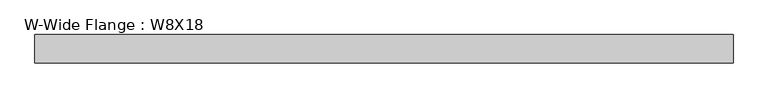
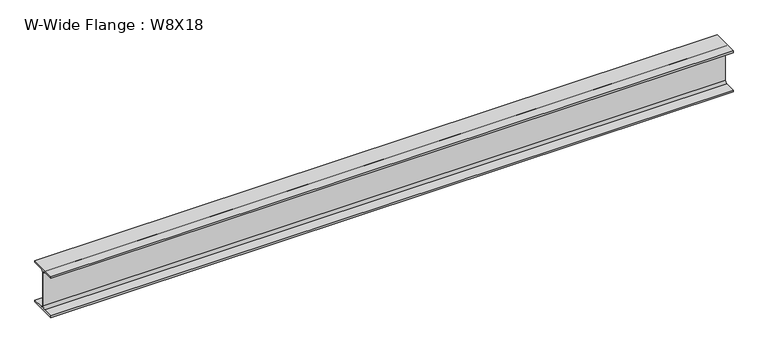
"""IFC4 building model written with IfcOpenShell, lengths in millimetres: beam geometry, W-Wide Flange : W8X18."""

from ifc_helpers import new_model, si_unit, point, frame, frame_2d, origin, place, context, project, spatial, polyline, circle_curve, trimmed, segment, composite_curve, outline, extrude, source, transform, mapped, element, save


def w_wide_flange_w8x18_c4c3ec7c(model_context):
    return source(origin(), model_context, "Body", "SweptSolid", [
        extrude(outline(composite_curve([segment(polyline([(66.675, -94.996), (66.675, -103.378), (-66.675, -103.378), (-66.675, -94.996), (-15.1765, -94.996)]), True, "CONTINUOUS"), segment(trimmed(circle_curve(frame_2d((-15.1765, -82.7405)), 12.2555), [point((-15.1765, -94.996))], [point((-2.921, -82.7405))], True, "CARTESIAN"), True, "CONTINUOUS"), segment(polyline([(-2.921, -82.7405), (-2.921, 82.7405)]), True, "CONTINUOUS"), segment(trimmed(circle_curve(frame_2d((-15.1765, 82.7405)), 12.2555), [point((-2.921, 82.7405))], [point((-15.1765, 94.996))], True, "CARTESIAN"), True, "CONTINUOUS"), segment(polyline([(-15.1765, 94.996), (-66.675, 94.996), (-66.675, 103.378), (66.675, 103.378), (66.675, 94.996), (15.1765, 94.996)]), True, "CONTINUOUS"), segment(trimmed(circle_curve(frame_2d((15.1765, 82.7405)), 12.2555), [point((15.1765, 94.996))], [point((2.921, 82.7405))], True, "CARTESIAN"), True, "CONTINUOUS"), segment(polyline([(2.921, 82.7405), (2.921, -82.7405)]), True, "CONTINUOUS"), segment(trimmed(circle_curve(frame_2d((15.1765, -82.7405)), 12.2555), [point((2.921, -82.7405))], [point((15.1765, -94.996))], True, "CARTESIAN"), True, "CONTINUOUS"), segment(polyline([(15.1765, -94.996), (66.675, -94.996)]), True, "CONTINUOUS")], self_intersect=False)), frame((-1531.8878906, 0.0, 0.0), z_axis=(1.0, 0.0, 0.0), x_axis=(0.0, 1.0, 0.0)), (0.0, 0.0, 1.0), 3263.6023437),
    ])


if __name__ == "__main__":
    model = new_model("IFC4")
    model_context = context("Model", 3, world=origin())
    ifc_project = project(units=[si_unit("LENGTHUNIT", "METRE", prefix="MILLI")], contexts=[model_context])
    site = spatial("IfcSite", under=ifc_project)
    building = spatial("IfcBuilding", under=site)
    placement = place(None, origin())
    w_wide_flange_w8x18_shape = w_wide_flange_w8x18_c4c3ec7c(model_context)
    element("IfcBeam", 1, ObjectType="W-Wide Flange : W8X18", at=placement, inside=building, context=model_context, shape_type="MappedRepresentation", body=[
        mapped(w_wide_flange_w8x18_shape, transform((0.0, 0.0, 0.0), x_axis=(1.0, 0.0, 0.0), y_axis=(0.0, 1.0, 0.0), z_axis=(0.0, 0.0, 1.0))),
    ])
    save(model, "model.ifc")

# Revit data of these elements
# Type "W-Wide Flange : W8X18"
#   Assembly Code = "B10"
#   W = 18
#   Length [instance default] = 1524 mm
#   bf = 133.35 mm
#   d = 206.756 mm
#   k = 20.638 mm
#   k2 = 12.256 mm
#   tf = 8.382 mm
#   tw = 5.842 mm
#   A = 0.00339354 m²
#   Structural Material [instance default] = Steel ASTM A992
# Element 1 (IfcBeam, "W-Wide Flange : W8X18")
#   Structural Material = Aluminum, Anodized Red
#   Materials on its faces: "Aluminum, Anodized Red"
# Materials
#   "Steel ASTM A992": class "Metal", colour RGB 128 0 0, transparency 0, Description = "Structural steel 50ksi", Cost = 0
#   "Aluminum, Anodized Red": class "Metal", colour RGB 120 120 120, transparency 0, Description = "Anodized aluminum, red", Cost = 0
